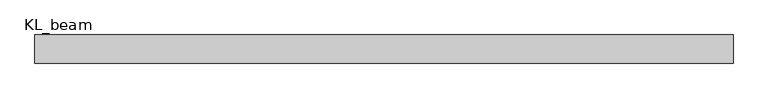
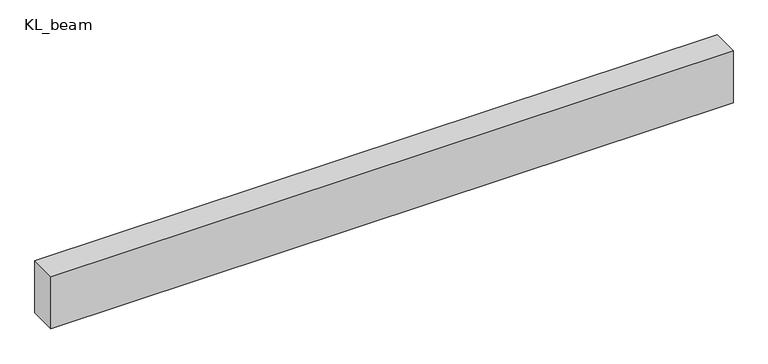
"""IFC4 building model written with IfcOpenShell, lengths in millimetres: beam geometry, 混凝土 - 矩形梁 : KL_beam."""

from ifc_helpers import new_model, si_unit, frame, origin, place, context, project, spatial, polyline, outline, extrude, source, transform, mapped, element, save


def kl_beam_4b589649(model_context):
    return source(origin(), model_context, "Body", "SweptSolid", [
        extrude(outline(polyline([(4962.0, 200.0), (4962.0, -200.0), (-4962.0, -200.0), (-4962.0, 200.0), (4962.0, 200.0)])), frame((0.0, 0.0, -400.0), z_axis=(0.0, 0.0, 1.0), x_axis=(1.0, 0.0, 0.0)), (0.0, 0.0, 1.0), 800.0),
    ])


if __name__ == "__main__":
    model = new_model("IFC4")
    model_context = context("Model", 3, world=origin())
    ifc_project = project(units=[si_unit("LENGTHUNIT", "METRE", prefix="MILLI")], contexts=[model_context])
    site = spatial("IfcSite", under=ifc_project)
    building = spatial("IfcBuilding", under=site)
    placement = place(None, origin())
    kl_beam_shape = kl_beam_4b589649(model_context)
    element("IfcBeam", 1, ObjectType="混凝土 - 矩形梁 : KL_beam", at=placement, inside=building, context=model_context, shape_type="MappedRepresentation", body=[
        mapped(kl_beam_shape, transform((0.0, 0.0, 0.0), x_axis=(1.0, 0.0, 0.0), y_axis=(0.0, 1.0, 0.0), z_axis=(0.0, 0.0, 1.0))),
    ])
    save(model, "model.ifc")

# Revit data of these elements
# Type "混凝土 - 矩形梁 : KL_beam"
#   Length [instance default] = 1524 mm
#   b = 400 mm
#   h = 800 mm
#   Structural Material [instance default] = 混凝土 - 现场浇注混凝土
#   Assembly Code = ""
# Element 1 (IfcBeam, "混凝土 - 矩形梁 : KL_beam")
#   Structural Material = none
# Materials
#   "混凝土 - 现场浇注混凝土": class "混凝土", colour RGB 192 192 192, transparency 0
